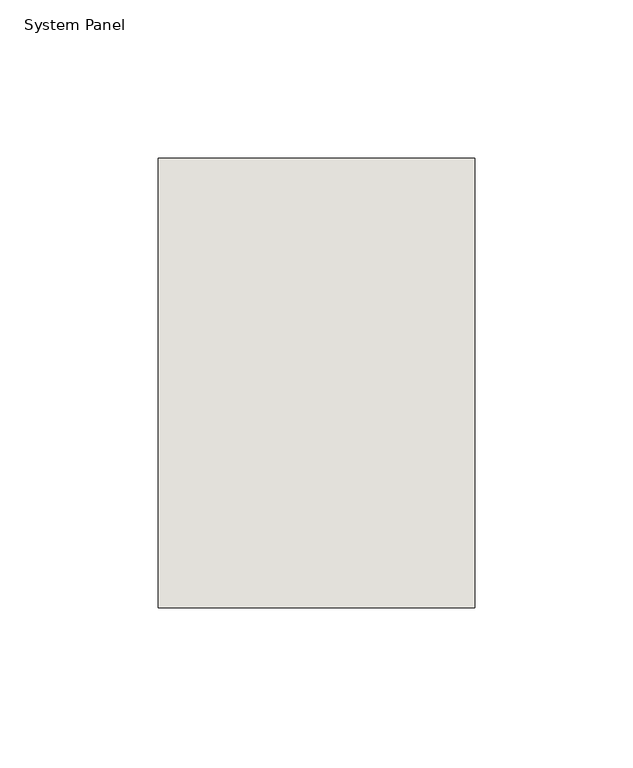
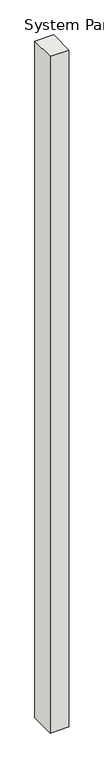
"""IFC4 building model written with IfcOpenShell, lengths in millimetres: wall geometry, System Panel : NLRS_21_CWP_hsb-vulling minerale wol 142 _gen_rsf."""

from ifc_helpers import new_model, si_unit, origin, origin_with_axes, place, context, project, spatial, polyline, outline, extrude, source, transform, mapped, element, save


def system_panel_45496c6a(model_context):
    return source(origin(), model_context, "Body", "SweptSolid", [
        extrude(outline(polyline([(49.9999998, -71.0), (-49.9999998, -71.0), (-49.9999998, 71.0), (49.9999998, 71.0), (49.9999998, -71.0)])), origin_with_axes(), (0.0, 0.0, 1.0), 3849.0),
    ])


if __name__ == "__main__":
    model = new_model("IFC4")
    model_context = context("Model", 3, world=origin())
    ifc_project = project(units=[si_unit("LENGTHUNIT", "METRE", prefix="MILLI")], contexts=[model_context])
    site = spatial("IfcSite", under=ifc_project)
    building = spatial("IfcBuilding", under=site)
    placement = place(None, origin())
    system_panel_shape = system_panel_45496c6a(model_context)
    element("IfcWall", 1, ObjectType="System Panel : NLRS_21_CWP_hsb-vulling minerale wol 142 _gen_rsf", at=placement, inside=building, context=model_context, shape_type="MappedRepresentation", body=[
        mapped(system_panel_shape, transform((0.0, 0.0, 0.0), x_axis=(1.0, 0.0, 0.0), y_axis=(0.0, 1.0, 0.0), z_axis=(0.0, 0.0, 1.0))),
    ])
    save(model, "model.ifc")

# Revit data of these elements
# Type "System Panel : NLRS_21_CWP_hsb-vulling minerale wol 142 _gen_rsf"
#   Type IfcGUID = "07M7mRoiH1CR8m_RSKIwpC"
#   Assembly Code = "21.23"
#   IfcExportAs = "IfcWall"
# Element 1 (IfcWall, "System Panel : NLRS_21_CWP_hsb-vulling minerale wol 142 _gen_rsf")
#   Materials on its faces: "NLRS_m1_isolatie minerale wol_gen_rsf"
# Materials
#   "NLRS_m1_isolatie minerale wol_gen_rsf": class "M - Anorganische materialen", colour RGB 200 200 140, transparency 0, Keynote = "m1", Manufacturer = "Revit Standards Foundation", URL = "www.revitstandards.org", Description = "isolatie minerale wol", Cost = 0
